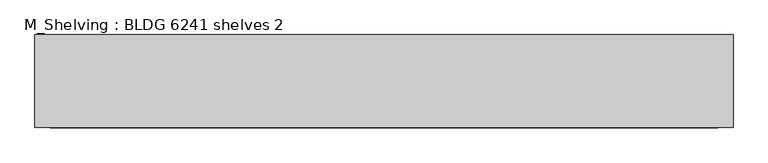
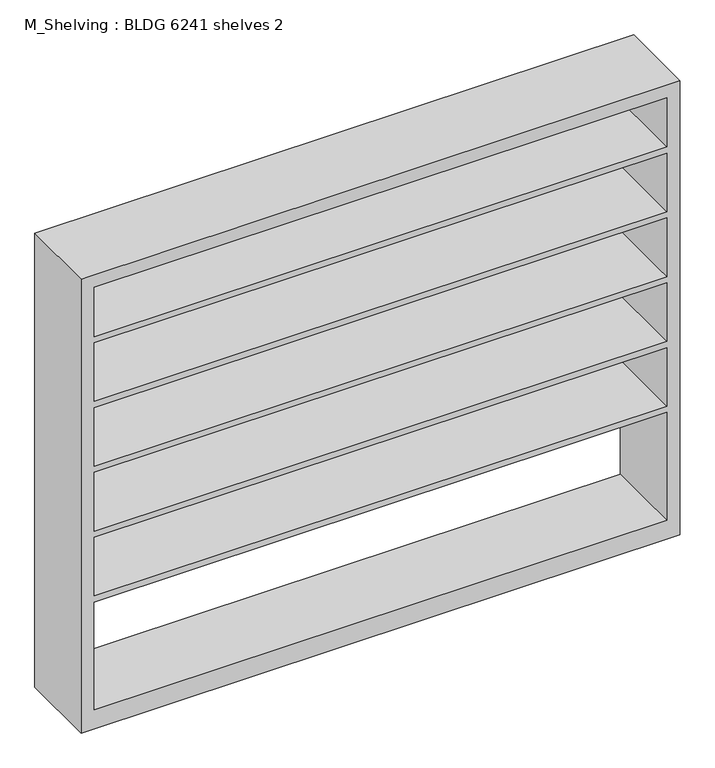
"""IFC4 building model written with IfcOpenShell, lengths in millimetres: furniture geometry, M_Shelving : BLDG 6241 shelves 2."""

from ifc_helpers import new_model, si_unit, frame, origin, place, context, project, spatial, polyline, outline, extrude, source, transform, mapped, element, save


def m_shelving_bldg_6241_shelves_2_ab080c00(model_context):
    return source(origin(), model_context, "Body", "SweptSolid", [
        extrude(outline(polyline([(0.0, 1143.0), (1830.0, 1143.0), (1830.0, -1143.0), (0.0, -1143.0), (0.0, 1143.0)]), holes=[polyline([(1779.2, 1092.2), (1581.2714286, 1092.2), (1581.2714286, -1092.2), (1779.2, -1092.2), (1779.2, 1092.2)]), polyline([(76.2, 1092.2), (76.2, -1092.2), (510.1571429, -1092.2), (510.1571429, 1092.2), (76.2, 1092.2)]), polyline([(1058.4142857, -1092.2), (1294.4428571, -1092.2), (1294.4428571, 1092.2), (1058.4142857, 1092.2), (1058.4142857, -1092.2)]), polyline([(1555.8714286, 1092.2), (1319.8428571, 1092.2), (1319.8428571, -1092.2), (1555.8714286, -1092.2), (1555.8714286, 1092.2)]), polyline([(1033.0142857, 1092.2), (796.9857143, 1092.2), (796.9857143, -1092.2), (1033.0142857, -1092.2), (1033.0142857, 1092.2)]), polyline([(771.5857143, 1092.2), (535.5571429, 1092.2), (535.5571429, -1092.2), (771.5857143, -1092.2), (771.5857143, 1092.2)])]), frame((0.0, -457.2, 0.0), z_axis=(0.0, 1.0, 0.0), x_axis=(0.0, 0.0, 1.0)), (0.0, 0.0, 1.0), 304.8),
    ])


if __name__ == "__main__":
    model = new_model("IFC4")
    model_context = context("Model", 3, world=origin())
    ifc_project = project(units=[si_unit("LENGTHUNIT", "METRE", prefix="MILLI")], contexts=[model_context])
    site = spatial("IfcSite", under=ifc_project)
    building = spatial("IfcBuilding", under=site)
    placement = place(None, origin())
    m_shelving_bldg_6241_shelves_2_shape = m_shelving_bldg_6241_shelves_2_ab080c00(model_context)
    element("IfcFurniture", 1, ObjectType="M_Shelving : BLDG 6241 shelves 2", at=placement, inside=building, context=model_context, shape_type="MappedRepresentation", body=[
        mapped(m_shelving_bldg_6241_shelves_2_shape, transform((0.0, 0.0, 0.0), x_axis=(1.0, 0.0, 0.0), y_axis=(0.0, 1.0, 0.0), z_axis=(0.0, 0.0, 1.0))),
    ])
    save(model, "model.ifc")

# Revit data of these elements
# Type "M_Shelving : BLDG 6241 shelves 2"
#   Depth = 1' - 0"
#   Height = 6' - 0.04724"
#   Width = 7' - 6"
#   Material = Birch
#   Default Elevation = 0
# Element 1 (IfcFurniture, "M_Shelving : BLDG 6241 shelves 2")
#   Materials on its faces: "Birch"
# Materials
#   "Birch": class "Wood", colour RGB 224 178 126, transparency 0, Description = "Betula Alleghaniensis", Cost = 0
